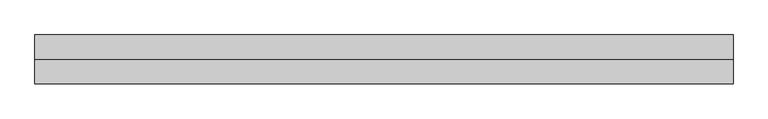
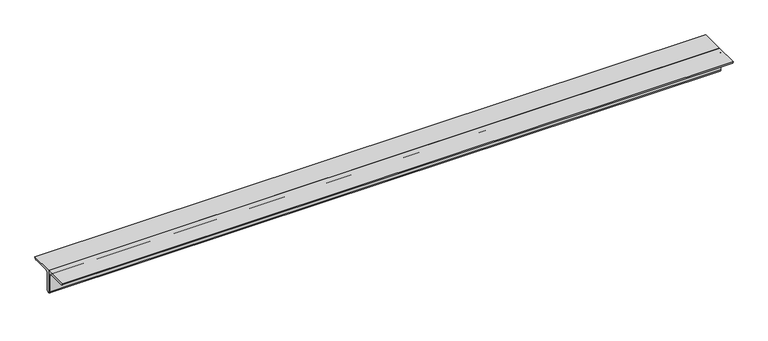
"""IFC4 building model written with IfcOpenShell, lengths in millimetres: member geometry, 0123_Steel Framing_2Ls-KSD3502 : H_SB_AR_S03_2Ls-130x130x12_HBR1."""

from ifc_helpers import new_model, si_unit, point, frame, frame_2d, origin, place, context, project, spatial, polyline, circle_curve, trimmed, segment, composite_curve, outline, extrude, source, transform, mapped, element, save


def member_1f5b8c5a(model_context):
    return source(origin(), model_context, "Body", "SweptSolid", [
        extrude(outline(composite_curve([segment(polyline([(0.0, 36.4), (130.0, 36.4)]), True, "CONTINUOUS"), segment(trimmed(circle_curve(frame_2d((118.0, 36.4)), 12.0), [point((130.0, 36.4))], [point((118.0, 24.4))], False, "CARTESIAN"), True, "CONTINUOUS"), segment(polyline([(118.0, 24.4), (24.0, 24.4)]), True, "CONTINUOUS"), segment(trimmed(circle_curve(frame_2d((24.0, 12.4)), 12.0), [point((24.0, 24.4))], [point((12.0, 12.4))], True, "CARTESIAN"), True, "CONTINUOUS"), segment(polyline([(12.0, 12.4), (12.0, -81.6)]), True, "CONTINUOUS"), segment(trimmed(circle_curve(frame_2d((0.0, -81.6)), 12.0), [point((12.0, -81.6))], [point((0.0, -93.6))], False, "CARTESIAN"), True, "CONTINUOUS"), segment(polyline([(0.0, -93.6), (0.0, 36.4)]), True, "CONTINUOUS")], self_intersect=False)), frame((-1844.6975967, 0.0, 0.0), z_axis=(1.0, 0.0, 0.0), x_axis=(0.0, 1.0, 0.0)), (0.0, 0.0, 1.0), 3701.6272171),
        extrude(outline(composite_curve([segment(polyline([(0.0, 36.4), (0.0, -93.6)]), True, "CONTINUOUS"), segment(trimmed(circle_curve(frame_2d((0.0, -81.6)), 12.0), [point((0.0, -93.6))], [point((-12.0, -81.6))], False, "CARTESIAN"), True, "CONTINUOUS"), segment(polyline([(-12.0, -81.6), (-12.0, 12.4)]), True, "CONTINUOUS"), segment(trimmed(circle_curve(frame_2d((-24.0, 12.4)), 12.0), [point((-12.0, 12.4))], [point((-24.0, 24.4))], True, "CARTESIAN"), True, "CONTINUOUS"), segment(polyline([(-24.0, 24.4), (-118.0, 24.4)]), True, "CONTINUOUS"), segment(trimmed(circle_curve(frame_2d((-118.0, 36.4)), 12.0), [point((-118.0, 24.4))], [point((-130.0, 36.4))], False, "CARTESIAN"), True, "CONTINUOUS"), segment(polyline([(-130.0, 36.4), (0.0, 36.4)]), True, "CONTINUOUS")], self_intersect=False)), frame((-1844.6975967, 0.0, 0.0), z_axis=(1.0, 0.0, 0.0), x_axis=(0.0, 1.0, 0.0)), (0.0, 0.0, 1.0), 3701.6272171),
    ])


if __name__ == "__main__":
    model = new_model("IFC4")
    model_context = context("Model", 3, world=origin())
    ifc_project = project(units=[si_unit("LENGTHUNIT", "METRE", prefix="MILLI")], contexts=[model_context])
    site = spatial("IfcSite", under=ifc_project)
    building = spatial("IfcBuilding", under=site)
    placement = place(None, origin())
    member_shape = member_1f5b8c5a(model_context)
    element("IfcMember", 1, ObjectType="0123_Steel Framing_2Ls-KSD3502 : H_SB_AR_S03_2Ls-130x130x12_HBR1", at=placement, inside=building, context=model_context, shape_type="MappedRepresentation", body=[
        mapped(member_shape, transform((0.0, 0.0, 0.0), x_axis=(1.0, 0.0, 0.0), y_axis=(0.0, 1.0, 0.0), z_axis=(0.0, 0.0, 1.0))),
    ])
    save(model, "model.ifc")

# Revit data of these elements
# Type "0123_Steel Framing_2Ls-KSD3502 : H_SB_AR_S03_2Ls-130x130x12_HBR1"
#   Assembly Code = "B10"
#   Legs = "SLBB"
#   W = 8.97
#   Perimeter = 1.04 m²/m
#   Nominal Weight = 46.80 kgf/m
#   Length [instance default] = 1000 mm
#   Space = 0 mm
#   b = 130 mm
#   d = 130 mm
#   t = 12 mm
#   y = 36.4 mm
#   A = 0.005952 m²
#   Structural Material [instance default] = Steel ASTM A36
# Element 1 (IfcMember, "0123_Steel Framing_2Ls-KSD3502 : H_SB_AR_S03_2Ls-130x130x12_HBR1")
#   Structural Material = Steel, 45-345
#   Materials on its faces: "Steel, 45-345"
# Materials
#   "Steel ASTM A36": class "Metal", colour RGB 199 199 199, transparency 0, Description = "Structural steel, ASTM A36 Grade B, mill finish", Cost = 0
#   "Steel, 45-345": class "Metal", colour RGB 189 187 185, transparency 0, Description = "Steel 345 MPa", Cost = 0
